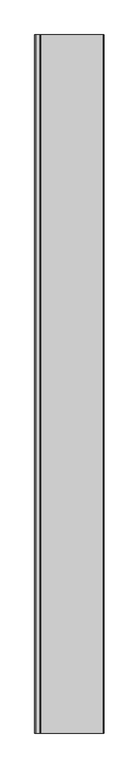
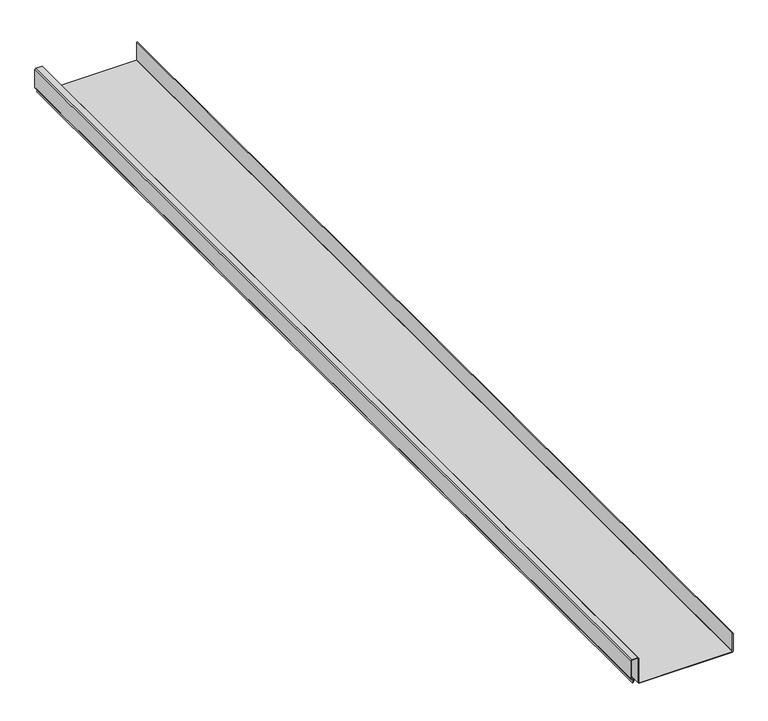
"""IFC4 building model written with IfcOpenShell, lengths in millimetres: proxy geometry, BEND PANEL1:BEND PANEL001:297518 : BEND PANEL1:BEND PANEL001:297518."""

import ifcopenshell
import ifcopenshell.guid

model = None  # the IFC model being written
_history = None  # IfcOwnerHistory: only IFC2X3 demands one
_inside = {}  # id of a spatial element -> (the spatial element, [elements in it])
_under = {}  # id of a project, library or spatial element -> (it, [spatial elements below it])
_declared = {}  # id of a project -> (the project, [libraries it declares])
_typed = {}  # id of a type object -> (the type object, [elements of that type])
_made_of = {}  # id of a material, layer set ... -> (it, [elements and type objects made of it])


def new_model(schema):
    """Start an empty IFC model of exactly this schema.

    Asked for "IFC4X3", IfcOpenShell would pick the latest addendum, in which some entities
    have other attributes; the version numbers below select the first issue.
    IFC2X3 requires an IfcOwnerHistory on every rooted entity: one is made here for all.
    """
    global model, _history
    if schema == "IFC4X3":
        model = ifcopenshell.file(schema_version=(4, 3, 0, 0))
    else:
        model = ifcopenshell.file(schema=schema)
    _inside.clear()
    _under.clear()
    _declared.clear()
    _typed.clear()
    _made_of.clear()
    _history = None
    if model.schema == "IFC2X3":
        org = make("IfcOrganization", Name="unknown")
        user = make(
            "IfcPersonAndOrganization",
            ThePerson=make("IfcPerson", FamilyName="unknown"),
            TheOrganization=org,
        )
        app = make(
            "IfcApplication",
            ApplicationDeveloper=org,
            Version="unknown",
            ApplicationFullName="unknown",
            ApplicationIdentifier="unknown",
        )
        _history = make(
            "IfcOwnerHistory",
            OwningUser=user,
            OwningApplication=app,
            ChangeAction="ADDED",
            CreationDate=0,
        )
    return model


def make(cls, **values):
    """One entity of the class cls with the attributes given. An attribute that is None is left unset."""
    return model.create_entity(
        cls, **{name: value for name, value in values.items() if value is not None}
    )


def rooted(cls, **values):
    """An entity with a GlobalId (a new one), such as an element, a storey or a relation."""
    return make(cls, GlobalId=ifcopenshell.guid.new(), OwnerHistory=_history, **values)


def si_unit(unit_type, name, prefix=None):
    """IfcSIUnit, for example si_unit("LENGTHUNIT", "METRE", prefix="MILLI")."""
    return make("IfcSIUnit", UnitType=unit_type, Prefix=prefix, Name=name)


def assignment(units):
    """IfcUnitAssignment: the units of a project."""
    return None if units is None else make("IfcUnitAssignment", Units=units)


def point(xyz):
    """IfcCartesianPoint."""
    return None if xyz is None else make("IfcCartesianPoint", Coordinates=xyz)


def direction(xyz):
    """IfcDirection."""
    return None if xyz is None else make("IfcDirection", DirectionRatios=xyz)


def frame(location, z_axis=None, x_axis=None):
    """IfcAxis2Placement3D, a coordinate frame: its origin and axes. An axis left out is left unset."""
    return make(
        "IfcAxis2Placement3D",
        Location=point(location),
        Axis=direction(z_axis),
        RefDirection=direction(x_axis),
    )


def origin():
    """The frame at (0, 0, 0) with its axes left unset."""
    return frame((0.0, 0.0, 0.0))


def place(relative_to, where):
    """IfcLocalPlacement: puts the frame where relative to a parent placement (None: the world)."""
    return make(
        "IfcLocalPlacement", PlacementRelTo=relative_to, RelativePlacement=where
    )


def context(
    kind, dimensions, precision=None, world=None, true_north=None, identifier=None
):
    """IfcGeometricRepresentationContext, for example the 3D "Model" context."""
    return make(
        "IfcGeometricRepresentationContext",
        ContextIdentifier=identifier,
        ContextType=kind,
        CoordinateSpaceDimension=dimensions,
        Precision=precision,
        WorldCoordinateSystem=world,
        TrueNorth=true_north,
    )


def project(units=None, contexts=None):
    """IfcProject with its units and contexts."""
    return rooted(
        "IfcProject",
        Name="project",
        RepresentationContexts=contexts,
        UnitsInContext=assignment(units),
    )


def spatial(cls, under=None, at=None, **own):
    """A site, building, storey or space (cls), placed at a placement, below another one or the project."""
    s = rooted(cls, ObjectPlacement=at, **own)
    if under is not None:
        _under.setdefault(under.id(), (under, []))[1].append(s)
    return s


def polyline(points):
    """IfcPolyline through the points."""
    return make("IfcPolyline", Points=[point(p) for p in points])


def outline(outer, holes=None, kind="AREA"):
    """IfcArbitraryClosedProfileDef: a profile drawn as a closed curve; with holes, ...WithVoids."""
    if holes is None:
        return make("IfcArbitraryClosedProfileDef", ProfileType=kind, OuterCurve=outer)
    return make(
        "IfcArbitraryProfileDefWithVoids",
        ProfileType=kind,
        OuterCurve=outer,
        InnerCurves=holes,
    )


def extrude(swept, where, along, depth):
    """IfcExtrudedAreaSolid: the profile swept, set in the frame where, extruded along a direction by depth."""
    return make(
        "IfcExtrudedAreaSolid",
        SweptArea=swept,
        Position=where,
        ExtrudedDirection=direction(along),
        Depth=depth,
    )


def shape(context_of_items, identifier, shape_type, items):
    """IfcShapeRepresentation: the items that make up one representation, for example the "Body"."""
    return make(
        "IfcShapeRepresentation",
        ContextOfItems=context_of_items,
        RepresentationIdentifier=identifier,
        RepresentationType=shape_type,
        Items=items,
    )


def source(mapping_origin, context_of_items, identifier, shape_type, items):
    """IfcRepresentationMap: a shape defined once, which mapped items show again and again."""
    return make(
        "IfcRepresentationMap",
        MappingOrigin=mapping_origin,
        MappedRepresentation=shape(context_of_items, identifier, shape_type, items),
    )


def transform(
    local_origin,
    x_axis=None,
    y_axis=None,
    z_axis=None,
    scale=None,
    scale2=None,
    scale3=None,
    uniform=True,
):
    """IfcCartesianTransformationOperator3D, or its non-uniform kind. x_axis, y_axis, z_axis: its Axis1, 2, 3."""
    if uniform:
        return make(
            "IfcCartesianTransformationOperator3D",
            Axis1=direction(x_axis),
            Axis2=direction(y_axis),
            LocalOrigin=point(local_origin),
            Scale=scale,
            Axis3=direction(z_axis),
        )
    return make(
        "IfcCartesianTransformationOperator3DnonUniform",
        Axis1=direction(x_axis),
        Axis2=direction(y_axis),
        LocalOrigin=point(local_origin),
        Scale=scale,
        Axis3=direction(z_axis),
        Scale2=scale2,
        Scale3=scale3,
    )


def mapped(mapping_source, mapping_target):
    """IfcMappedItem: shows the shape of a source again, moved by a transform."""
    return make(
        "IfcMappedItem", MappingSource=mapping_source, MappingTarget=mapping_target
    )


def made_of(thing, what):
    """Note that an element or type object is made of a material, layer set ...; save() writes the relation."""
    if what is not None:
        _made_of.setdefault(what.id(), (what, []))[1].append(thing)
    return thing


def element(
    cls,
    number,
    at=None,
    inside=None,
    cuts=None,
    type_object=None,
    material=None,
    context=None,
    identifier="Body",
    shape_type=None,
    held_by="IfcProductDefinitionShape",
    body=None,
    shapes=None,
    **own,
):
    """One element of the class cls, such as IfcWall. Its Tag is "e" and its number.

    at: its placement. inside: the storey or other place that contains it. cuts: it is an
    opening in that element (IfcRelVoidsElement). A single representation is given by context,
    identifier, shape_type and body (its items); several are given by shapes. held_by: the class
    of the entity that holds the representations. save() writes the other relations.
    """
    e = rooted(cls, Tag="e%d" % number, ObjectPlacement=at, **own)
    if body is not None:
        shapes = [shape(context, identifier, shape_type, body)]
    if shapes is not None:
        e.Representation = make(held_by, Representations=shapes)
    if inside is not None:
        _inside.setdefault(inside.id(), (inside, []))[1].append(e)
    if cuts is not None:
        rooted(
            "IfcRelVoidsElement", RelatingBuildingElement=cuts, RelatedOpeningElement=e
        )
    if type_object is not None:
        _typed.setdefault(type_object.id(), (type_object, []))[1].append(e)
    return made_of(e, material)


def aggregate(whole, parts):
    """IfcRelAggregates: a whole, such as a stair, and the parts it consists of."""
    return rooted("IfcRelAggregates", RelatingObject=whole, RelatedObjects=parts)


def save(model, path):
    """Write the relations noted so far, then the file.

    IfcRelAggregates (storeys below a building ...), IfcRelContainedInSpatialStructure (elements
    in a storey), IfcRelDefinesByType, IfcRelAssociatesMaterial and IfcRelDeclares: one each for
    every whole, place, type object, material and project.
    """
    for whole, parts in _under.values():
        aggregate(whole, parts)
    for where, things in _inside.values():
        rooted(
            "IfcRelContainedInSpatialStructure",
            RelatedElements=things,
            RelatingStructure=where,
        )
    for kind, things in _typed.values():
        rooted("IfcRelDefinesByType", RelatedObjects=things, RelatingType=kind)
    for what, things in _made_of.values():
        rooted("IfcRelAssociatesMaterial", RelatedObjects=things, RelatingMaterial=what)
    for by, libraries in _declared.values():
        rooted("IfcRelDeclares", RelatingContext=by, RelatedDefinitions=libraries)
    model.write(path)


def generic_models_3c4cd455(model_context):
    return source(origin(), model_context, "Body", "SweptSolid", [
        extrude(outline(polyline([(42594.4082245, 10627.268636), (42589.7865091, 10625.1134947), (42589.2833292, 10626.1925674), (42594.3520112, 10628.5561327), (42596.210073, 10627.8798535), (42598.2005361, 10623.6113437), (42599.4643694, 10622.8111715), (42634.8859537, 10622.8111715), (42636.2841216, 10624.2093394), (42636.2841216, 10634.9075309), (42634.8859537, 10636.3056988), (42585.9088212, 10636.3056988), (42584.5106533, 10637.7038667), (42584.5106533, 10818.8468367), (42585.9101309, 10820.2463143), (42623.1706509, 10820.2463143), (42623.1706509, 10819.0556893), (42586.4033039, 10819.0556893), (42585.7012783, 10818.3536636), (42585.7012783, 10638.1970397), (42586.4019942, 10637.4963238), (42635.3791267, 10637.4963238), (42637.4747466, 10635.4007039), (42637.4747466, 10623.7161664), (42635.3791267, 10621.6205465), (42599.1191461, 10621.6205465), (42597.268896, 10622.7919974), (42595.3394273, 10626.9297059), (42594.4082245, 10627.268636)])), frame((0.0, -774.5581163, 0.0), z_axis=(0.0, 1.0, 0.0), x_axis=(0.0, 0.0, 1.0)), (0.0, 0.0, 1.0), 1999.85),
    ])


if __name__ == "__main__":
    model = new_model("IFC4")
    model_context = context("Model", 3, world=origin())
    ifc_project = project(units=[si_unit("LENGTHUNIT", "METRE", prefix="MILLI")], contexts=[model_context])
    site = spatial("IfcSite", under=ifc_project)
    building = spatial("IfcBuilding", under=site)
    placement = place(None, origin())
    generic_models_shape = generic_models_3c4cd455(model_context)
    element("IfcBuildingElementProxy", 1, Name="BEND PANEL1:BEND PANEL001:297518 : BEND PANEL1:BEND PANEL001:297518", ObjectType="BEND PANEL1:BEND PANEL001:297518 : BEND PANEL1:BEND PANEL001:297518", at=placement, inside=building, context=model_context, shape_type="MappedRepresentation", body=[
        mapped(generic_models_shape, transform((0.0, 0.0, 0.0), x_axis=(1.0, 0.0, 0.0), y_axis=(0.0, 1.0, 0.0), z_axis=(0.0, 0.0, 1.0))),
    ])
    save(model, "model.ifc")

# Revit data of these elements
# Type "BEND PANEL1:BEND PANEL001:297518 : BEND PANEL1:BEND PANEL001:297518"
#   NameOverride = "BEND PANEL1:BEND PANEL001:297518"
#   ObjectTypeOverride = "BEND PANEL1:BEND PANEL001"
#   Reference = "BEND PANEL001"
#   Category = "Generic Models"
#   Tag = "297518"
# Element 1 (IfcBuildingElementProxy, "BEND PANEL1:BEND PANEL001:297518 : BEND PANEL1:BEND PANEL001:297518")
#   Materials on its faces: "STANDING SEAM METAL ROOF FOLLOW MANU. RECOMMENDED EDGE/TRANSITION DETAILS"
# Materials
#   "STANDING SEAM METAL ROOF FOLLOW MANU. RECOMMENDED EDGE/TRANSITION DETAILS": class "Unassigned", colour RGB 128 128 128, transparency 0, Cost = 0
